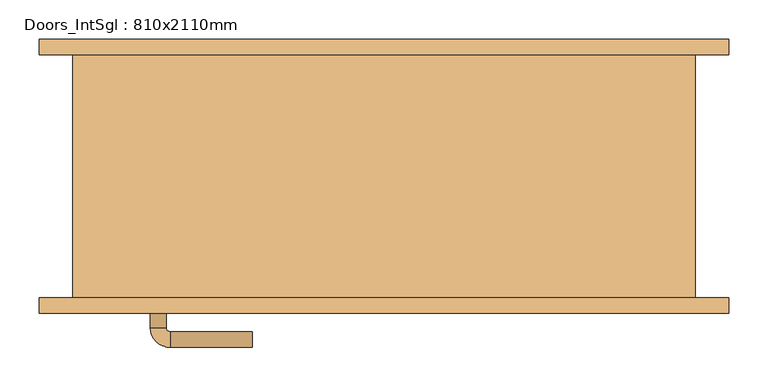
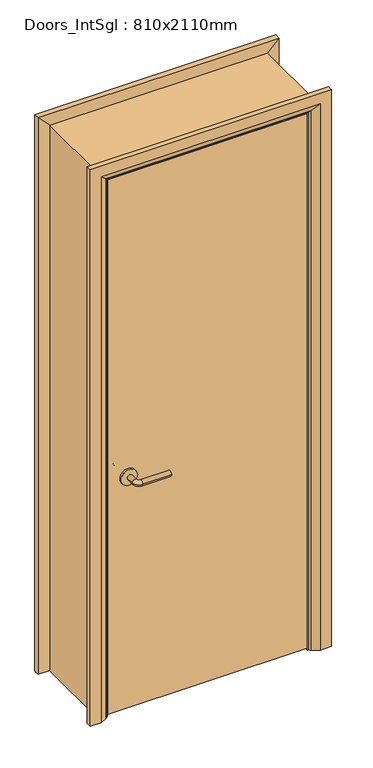
"""IFC4 building model written with IfcOpenShell, lengths in millimetres: door geometry, Doors_IntSgl : 810x2110mm."""

from ifc_helpers import new_model, si_unit, point, frame, frame_2d, origin, place, context, project, spatial, polyline, circle_curve, ellipse_curve, trimmed, segment, composite_curve, outline, extrude, faceted_brep, source, transform, mapped, element, save
from ifc_brep_helpers import plane_surface, cylinder_surface, revolved_surface, advanced_brep


def doors_intsgl_810x2110mm_eeb1298a(model_context):
    return source(origin(), model_context, "Body", "SolidModel", [
        advanced_brep(
        [(-298.0, -109.0, 900.0), (-278.0, -109.0, 900.0), (-298.0, -79.0, 900.0), (-278.0, -79.0, 900.0), (-273.0, -74.0, 900.0), (-273.0, -54.0, 900.0), (-168.0, -54.0, 900.0), (-168.0, -74.0, 900.0)],
        [
            (0, 1, circle_curve(frame((-288.0, -109.0, 900.0), z_axis=(0.0, -1.0, 0.0), x_axis=(1.0, 0.0, 0.0)), 10.0)),
            (1, 0, circle_curve(frame((-288.0, -109.0, 900.0), z_axis=(0.0, -1.0, 0.0), x_axis=(1.0, 0.0, 0.0)), 10.0)),
            (0, 2),
            (2, 3, circle_curve(frame((-288.0, -79.0, 900.0), z_axis=(0.0, -1.0, 0.0), x_axis=(1.0, 0.0, 0.0)), 10.0)),
            (3, 1),
            (3, 2, circle_curve(frame((-288.0, -79.0, 900.0), z_axis=(0.0, -1.0, 0.0), x_axis=(1.0, 0.0, 0.0)), 10.0)),
            (4, 3, circle_curve(frame((-273.0, -79.0, 900.0), z_axis=(0.0, 0.0, 1.0), x_axis=(-1.0, 0.0, 0.0)), 5.0)),
            (2, 5, circle_curve(frame((-273.0, -79.0, 900.0), z_axis=(0.0, 0.0, -1.0), x_axis=(-1.0, 0.0, 0.0)), 25.0)),
            (5, 4, circle_curve(frame((-273.0, -64.0, 900.0), z_axis=(-1.0, 0.0, 0.0), x_axis=(0.0, -1.0, 0.0)), 10.0)),
            (4, 5, circle_curve(frame((-273.0, -64.0, 900.0), z_axis=(-1.0, 0.0, 0.0), x_axis=(0.0, -1.0, 0.0)), 10.0)),
            (6, 7, circle_curve(frame((-168.0, -64.0, 900.0), z_axis=(1.0, 0.0, 0.0), x_axis=(0.0, -1.0, 0.0)), 10.0)),
            (7, 6, circle_curve(frame((-168.0, -64.0, 900.0), z_axis=(1.0, 0.0, 0.0), x_axis=(0.0, -1.0, 0.0)), 10.0)),
            (5, 6),
            (7, 4),
        ],
        [
            plane_surface(frame((-288.0, -109.0, 900.0), z_axis=(0.0, -1.0, 0.0), x_axis=(0.0, 0.0, 1.0))),
            cylinder_surface(frame((-288.0, -109.0, 900.0), z_axis=(0.0, -1.0, 0.0), x_axis=(1.0, 0.0, 0.0)), 10.0),
            revolved_surface(trimmed(ellipse_curve(frame((-288.0, -79.0, 900.0), z_axis=(0.0, -1.0, 0.0), x_axis=(1.0, 0.0, 0.0)), 10.0, 10.0), [point((-298.0, -79.0, 900.0))], [point((-278.0, -79.0, 900.0))], True, "CARTESIAN"), (-273.0, -79.0, 900.0), (0.0, 0.0, -1.0)),
            revolved_surface(trimmed(ellipse_curve(frame((-288.0, -79.0, 900.0), z_axis=(0.0, -1.0, 0.0), x_axis=(1.0, 0.0, 0.0)), 10.0, 10.0), [point((-278.0, -79.0, 900.0))], [point((-298.0, -79.0, 900.0))], True, "CARTESIAN"), (-273.0, -79.0, 900.0), (0.0, 0.0, -1.0)),
            plane_surface(frame((-168.0, -64.0, 900.0), z_axis=(1.0, 0.0, 0.0), x_axis=(0.0, 0.0, 1.0))),
            cylinder_surface(frame((-273.0, -64.0, 900.0), z_axis=(-1.0, 0.0, 0.0), x_axis=(0.0, -1.0, 0.0)), 10.0),
        ],
        [
            (0, [[1, 2]]),
            (1, [[-1, 3, 4, 5]]),
            (1, [[-2, -5, 6, -3]]),
            (2, [[7, -4, 8, 9]]),
            (3, [[-8, -6, -7, 10]]),
            (4, [[11, 12]]),
            (5, [[-9, 13, -12, 14]]),
            (5, [[-10, -14, -11, -13]]),
        ],
    ),
        extrude(outline(composite_curve([segment(trimmed(circle_curve(frame_2d((900.0, -290.5)), 30.0), [point((900.0, -320.5))], [point((900.0, -260.5))], False, "CARTESIAN"), True, "CONTINUOUS"), segment(trimmed(circle_curve(frame_2d((900.0, -290.5)), 30.0), [point((900.0, -260.5))], [point((900.0, -320.5))], False, "CARTESIAN"), True, "CONTINUOUS")], self_intersect=False)), frame((0.0, -117.0, 0.0), z_axis=(0.0, 1.0, 0.0), x_axis=(0.0, 0.0, 1.0)), (0.0, 0.0, 1.0), 8.0),
        advanced_brep(
        [(-298.0, -163.0, 900.0), (-278.0, -163.0, 900.0), (-278.0, -193.0, 900.0), (-298.0, -193.0, 900.0), (-273.0, -198.0, 900.0), (-273.0, -218.0, 900.0), (-168.0, -218.0, 900.0), (-168.0, -198.0, 900.0)],
        [
            (0, 1, circle_curve(frame((-288.0, -163.0, 900.0), z_axis=(0.0, 1.0, 0.0), x_axis=(1.0, 0.0, 0.0)), 10.0)),
            (1, 0, circle_curve(frame((-288.0, -163.0, 900.0), z_axis=(0.0, 1.0, 0.0), x_axis=(1.0, 0.0, 0.0)), 10.0)),
            (1, 2),
            (2, 3, circle_curve(frame((-288.0, -193.0, 900.0), z_axis=(0.0, 1.0, 0.0), x_axis=(1.0, 0.0, 0.0)), 10.0)),
            (3, 0),
            (3, 2, circle_curve(frame((-288.0, -193.0, 900.0), z_axis=(0.0, 1.0, 0.0), x_axis=(1.0, 0.0, 0.0)), 10.0)),
            (4, 5, circle_curve(frame((-273.0, -208.0, 900.0), z_axis=(-1.0, 0.0, 0.0), x_axis=(0.0, 1.0, 0.0)), 10.0)),
            (5, 3, circle_curve(frame((-273.0, -193.0, 900.0), z_axis=(0.0, 0.0, -1.0), x_axis=(-1.0, 0.0, 0.0)), 25.0)),
            (2, 4, circle_curve(frame((-273.0, -193.0, 900.0), z_axis=(0.0, 0.0, 1.0), x_axis=(-1.0, 0.0, 0.0)), 5.0)),
            (5, 4, circle_curve(frame((-273.0, -208.0, 900.0), z_axis=(-1.0, 0.0, 0.0), x_axis=(0.0, 1.0, 0.0)), 10.0)),
            (6, 7, circle_curve(frame((-168.0, -208.0, 900.0), z_axis=(1.0, 0.0, 0.0), x_axis=(0.0, 1.0, 0.0)), 10.0)),
            (7, 6, circle_curve(frame((-168.0, -208.0, 900.0), z_axis=(1.0, 0.0, 0.0), x_axis=(0.0, 1.0, 0.0)), 10.0)),
            (4, 7),
            (6, 5),
        ],
        [
            plane_surface(frame((-288.0, -163.0, 900.0), z_axis=(0.0, 1.0, 0.0), x_axis=(0.0, 0.0, 1.0))),
            cylinder_surface(frame((-288.0, -163.0, 900.0), z_axis=(0.0, 1.0, 0.0), x_axis=(1.0, 0.0, 0.0)), 10.0),
            revolved_surface(trimmed(ellipse_curve(frame((-288.0, -193.0, 900.0), z_axis=(0.0, -1.0, 0.0), x_axis=(1.0, 0.0, 0.0)), 10.0, 10.0), [point((-298.0, -193.0, 900.0))], [point((-278.0, -193.0, 900.0))], True, "CARTESIAN"), (-273.0, -193.0, 900.0), (0.0, 0.0, -1.0)),
            revolved_surface(trimmed(ellipse_curve(frame((-288.0, -193.0, 900.0), z_axis=(0.0, -1.0, 0.0), x_axis=(1.0, 0.0, 0.0)), 10.0, 10.0), [point((-278.0, -193.0, 900.0))], [point((-298.0, -193.0, 900.0))], True, "CARTESIAN"), (-273.0, -193.0, 900.0), (0.0, 0.0, -1.0)),
            plane_surface(frame((-168.0, -208.0, 900.0), z_axis=(1.0, 0.0, 0.0), x_axis=(0.0, 0.0, 1.0))),
            cylinder_surface(frame((-273.0, -208.0, 900.0), z_axis=(-1.0, 0.0, 0.0), x_axis=(0.0, 1.0, 0.0)), 10.0),
        ],
        [
            (0, [[1, 2]]),
            (1, [[3, 4, 5, -2]]),
            (1, [[-5, 6, -3, -1]]),
            (2, [[7, 8, -4, 9]]),
            (3, [[10, -9, -6, -8]]),
            (4, [[11, 12]]),
            (5, [[13, -11, 14, -7]]),
            (5, [[-14, -12, -13, -10]]),
        ],
    ),
        extrude(outline(composite_curve([segment(trimmed(circle_curve(frame_2d((900.0, -290.5)), 30.0), [point((900.0, -320.5))], [point((900.0, -260.5))], False, "CARTESIAN"), True, "CONTINUOUS"), segment(trimmed(circle_curve(frame_2d((900.0, -290.5)), 30.0), [point((900.0, -260.5))], [point((900.0, -320.5))], False, "CARTESIAN"), True, "CONTINUOUS")], self_intersect=False)), frame((0.0, -163.0, 0.0), z_axis=(0.0, 1.0, 0.0), x_axis=(0.0, 0.0, 1.0)), (0.0, 0.0, 1.0), 8.0),
        extrude(outline(polyline([(363.0, -117.0), (363.0, -155.0), (-363.0, -155.0), (-363.0, -117.0), (363.0, -117.0)])), frame((0.0, 0.0, 8.0), z_axis=(0.0, 0.0, 1.0), x_axis=(1.0, 0.0, 0.0)), (0.0, 0.0, 1.0), 2060.0),
        advanced_brep(
        [(440.0, -175.0, 0.0), (400.0, -175.0, 0.0), (374.0, -161.0, 0.0), (370.0, -155.0, 0.0), (440.0, -155.0, 0.0), (440.0, -155.0, 2145.0), (440.0, -175.0, 2145.0), (370.0, -155.0, 2075.0), (-370.0, -155.0, 2075.0), (-370.0, -155.0, 0.0), (-440.0, -155.0, 0.0), (-440.0, -155.0, 2145.0), (374.0, -161.0, 2079.0), (400.0, -175.0, 2105.0), (-440.0, -175.0, 2145.0), (-440.0, -175.0, 0.0), (-400.0, -175.0, 0.0), (-400.0, -175.0, 2105.0), (-374.0, -161.0, 2079.0), (-374.0, -161.0, 0.0)],
        [
            (0, 1),
            (1, 2),
            (2, 3, circle_curve(frame((378.0, -154.0, 0.0), z_axis=(0.0, 0.0, -1.0), x_axis=(1.0, 0.0, 0.0)), 8.0622577)),
            (3, 4),
            (4, 0),
            (4, 5),
            (5, 6),
            (6, 0),
            (3, 7),
            (7, 8),
            (8, 9),
            (9, 10),
            (10, 11),
            (11, 5),
            (2, 12),
            (12, 7, ellipse_curve(frame((378.0, -154.0, 2083.0), z_axis=(0.7071067811865475, 0.0, -0.7071067811865475), x_axis=(-0.7071067811865474, 0.0, -0.7071067811865476)), 11.4017543, 8.0622577)),
            (1, 13),
            (13, 12),
            (6, 14),
            (14, 15),
            (15, 16),
            (16, 17),
            (17, 13),
            (11, 14),
            (12, 18),
            (18, 8, ellipse_curve(frame((-378.0, -154.0, 2083.0), z_axis=(0.7071067811865475, 0.0, 0.7071067811865475), x_axis=(0.7071067811865476, 0.0, -0.7071067811865474)), 11.4017543, 8.0622577)),
            (17, 18),
            (15, 10),
            (9, 19, circle_curve(frame((-378.0, -154.0, 0.0), z_axis=(0.0, 0.0, -1.0), x_axis=(-1.0, 0.0, 0.0)), 8.0622577)),
            (19, 16),
            (18, 19),
        ],
        [
            plane_surface(frame((370.0, -155.0, 0.0), z_axis=(0.0, 0.0, -1.0), x_axis=(0.0, 1.0, 0.0))),
            plane_surface(frame((440.0, -175.0, 0.0), z_axis=(1.0, 0.0, 0.0), x_axis=(0.0, 0.0, 1.0))),
            plane_surface(frame((440.0, -155.0, 0.0), z_axis=(0.0, 1.0, 0.0), x_axis=(0.0, 0.0, 1.0))),
            cylinder_surface(frame((378.0, -154.0, 0.0), z_axis=(0.0, 0.0, -1.0), x_axis=(1.0, 0.0, 0.0)), 8.0622577),
            plane_surface(frame((374.0, -161.0, 0.0), z_axis=(-0.4740998230350126, -0.880471099922178, 0.0), x_axis=(0.0, 0.0, 1.0))),
            plane_surface(frame((400.0, -175.0, 0.0), z_axis=(0.0, -1.0, 0.0), x_axis=(0.0, 0.0, 1.0))),
            plane_surface(frame((440.0, -175.0, 2145.0), z_axis=(0.0, 0.0, 1.0), x_axis=(-1.0, 0.0, 0.0))),
            cylinder_surface(frame((370.0, -154.0, 2083.0), z_axis=(1.0, 0.0, 0.0), x_axis=(0.0, 0.0, 1.0)), 8.0622577),
            plane_surface(frame((374.0, -161.0, 2079.0), z_axis=(0.0, -0.8804710999221764, -0.4740998230350154), x_axis=(-1.0, 0.0, 0.0))),
            plane_surface(frame((-370.0, -155.0, 0.0), z_axis=(0.0, 0.0, -1.0), x_axis=(0.0, 1.0, 0.0))),
            plane_surface(frame((-440.0, -175.0, 2145.0), z_axis=(-1.0, 0.0, 0.0), x_axis=(0.0, 0.0, -1.0))),
            cylinder_surface(frame((-378.0, -154.0, 2075.0), z_axis=(0.0, 0.0, 1.0), x_axis=(-1.0, 0.0, 0.0)), 8.0622577),
            plane_surface(frame((-374.0, -161.0, 2079.0), z_axis=(0.47409982303501824, -0.8804710999221749, 0.0), x_axis=(0.0, 0.0, -1.0))),
        ],
        [
            (0, [[1, 2, 3, 4, 5]]),
            (1, [[6, 7, 8, -5]]),
            (2, [[9, 10, 11, 12, 13, 14, -6, -4]]),
            (3, [[15, 16, -9, -3]]),
            (4, [[17, 18, -15, -2]]),
            (5, [[-8, 19, 20, 21, 22, 23, -17, -1]]),
            (6, [[-14, 24, -19, -7]]),
            (7, [[25, 26, -10, -16]]),
            (8, [[-23, 27, -25, -18]]),
            (9, [[28, -12, 29, 30, -21]]),
            (10, [[-13, -28, -20, -24]]),
            (11, [[31, -29, -11, -26]]),
            (12, [[-22, -30, -31, -27]]),
        ],
    ),
        extrude(outline(polyline([(0.0, -346.0), (2051.0, -346.0), (2051.0, 346.0), (0.0, 346.0), (0.0, 365.0), (2070.0, 365.0), (2070.0, -365.0), (0.0, -365.0), (0.0, -346.0)])), frame((0.0, -115.0, 0.0), z_axis=(0.0, 1.0, 0.0), x_axis=(0.0, 0.0, 1.0)), (0.0, 0.0, 1.0), 32.0),
        advanced_brep(
        [(-440.0, 175.0, 0.0), (-400.0, 175.0, 0.0), (-374.0, 161.0, 0.0), (-370.0, 155.0, 0.0), (-440.0, 155.0, 0.0), (-440.0, 155.0, 2145.0), (-440.0, 175.0, 2145.0), (-370.0, 155.0, 2075.0), (-374.0, 161.0, 2079.0), (-400.0, 175.0, 2105.0), (440.0, 155.0, 2145.0), (440.0, 175.0, 2145.0), (370.0, 155.0, 2075.0), (374.0, 161.0, 2079.0), (400.0, 175.0, 2105.0), (440.0, 175.0, 0.0), (440.0, 155.0, 0.0), (370.0, 155.0, 0.0), (374.0, 161.0, 0.0), (400.0, 175.0, 0.0)],
        [
            (0, 1),
            (1, 2),
            (2, 3, circle_curve(frame((-378.0, 154.0, 0.0), z_axis=(0.0, 0.0, -1.0), x_axis=(-1.0, 0.0, 0.0)), 8.0622577)),
            (3, 4),
            (4, 0),
            (4, 5),
            (5, 6),
            (6, 0),
            (3, 7),
            (7, 5),
            (2, 8),
            (8, 7, ellipse_curve(frame((-378.0, 154.0, 2083.0), z_axis=(-0.7071067811865475, 0.0, -0.7071067811865475), x_axis=(0.7071067811865474, 0.0, -0.7071067811865476)), 11.4017543, 8.0622577)),
            (1, 9),
            (9, 8),
            (6, 9),
            (5, 10),
            (10, 11),
            (11, 6),
            (7, 12),
            (12, 10),
            (8, 13),
            (13, 12, ellipse_curve(frame((378.0, 154.0, 2083.0), z_axis=(-0.7071067811865475, 0.0, 0.7071067811865475), x_axis=(-0.7071067811865476, 0.0, -0.7071067811865474)), 11.4017543, 8.0622577)),
            (9, 14),
            (14, 13),
            (11, 14),
            (15, 16),
            (16, 17),
            (17, 18, circle_curve(frame((378.0, 154.0, 0.0), z_axis=(0.0, 0.0, -1.0), x_axis=(1.0, 0.0, 0.0)), 8.0622577)),
            (18, 19),
            (19, 15),
            (10, 16),
            (15, 11),
            (12, 17),
            (13, 18),
            (14, 19),
        ],
        [
            plane_surface(frame((-370.0, 227.8010989, 0.0), z_axis=(0.0, 0.0, -1.0), x_axis=(1.0, 0.0, 0.0))),
            plane_surface(frame((-440.0, 175.0, 0.0), z_axis=(-1.0, 0.0, 0.0), x_axis=(0.0, 0.0, 1.0))),
            plane_surface(frame((-440.0, 155.0, 0.0), z_axis=(0.0, -1.0, 0.0), x_axis=(0.0, 0.0, 1.0))),
            cylinder_surface(frame((-378.0, 154.0, 0.0), z_axis=(0.0, 0.0, -1.0), x_axis=(-1.0, 0.0, 0.0)), 8.0622577),
            plane_surface(frame((-374.0, 161.0, 0.0), z_axis=(0.4740998230350183, 0.8804710999221749, 0.0), x_axis=(0.0, 0.0, 1.0))),
            plane_surface(frame((-400.0, 175.0, 0.0), z_axis=(0.0, 1.0, 0.0), x_axis=(0.0, 0.0, 1.0))),
            plane_surface(frame((-440.0, 175.0, 2145.0), z_axis=(0.0, 0.0, 1.0), x_axis=(1.0, 0.0, 0.0))),
            plane_surface(frame((-440.0, 155.0, 2145.0), z_axis=(0.0, -1.0, 0.0), x_axis=(1.0, 0.0, 0.0))),
            cylinder_surface(frame((-370.0, 154.0, 2083.0), z_axis=(-1.0, 0.0, 0.0), x_axis=(0.0, 0.0, 1.0)), 8.0622577),
            plane_surface(frame((-374.0, 161.0, 2079.0), z_axis=(0.0, 0.8804710999221749, -0.4740998230350183), x_axis=(1.0, 0.0, 0.0))),
            plane_surface(frame((-400.0, 175.0, 2105.0), z_axis=(0.0, 1.0, 0.0), x_axis=(1.0, 0.0, 0.0))),
            plane_surface(frame((370.0, 227.8010989, 0.0), z_axis=(0.0, 0.0, -1.0), x_axis=(-1.0, 0.0, 0.0))),
            plane_surface(frame((440.0, 175.0, 2145.0), z_axis=(1.0, 0.0, 0.0), x_axis=(0.0, 0.0, -1.0))),
            plane_surface(frame((440.0, 155.0, 2145.0), z_axis=(0.0, -1.0, 0.0), x_axis=(0.0, 0.0, -1.0))),
            cylinder_surface(frame((378.0, 154.0, 2075.0), z_axis=(0.0, 0.0, 1.0), x_axis=(1.0, 0.0, 0.0)), 8.0622577),
            plane_surface(frame((374.0, 161.0, 2079.0), z_axis=(-0.4740998230350183, 0.8804710999221749, 0.0), x_axis=(0.0, 0.0, -1.0))),
            plane_surface(frame((400.0, 175.0, 2105.0), z_axis=(0.0, 1.0, 0.0), x_axis=(0.0, 0.0, -1.0))),
        ],
        [
            (0, [[1, 2, 3, 4, 5]]),
            (1, [[6, 7, 8, -5]]),
            (2, [[9, 10, -6, -4]]),
            (3, [[11, 12, -9, -3]]),
            (4, [[13, 14, -11, -2]]),
            (5, [[-8, 15, -13, -1]]),
            (6, [[16, 17, 18, -7]]),
            (7, [[19, 20, -16, -10]]),
            (8, [[21, 22, -19, -12]]),
            (9, [[23, 24, -21, -14]]),
            (10, [[-18, 25, -23, -15]]),
            (11, [[26, 27, 28, 29, 30]]),
            (12, [[31, -26, 32, -17]]),
            (13, [[33, -27, -31, -20]]),
            (14, [[34, -28, -33, -22]]),
            (15, [[35, -29, -34, -24]]),
            (16, [[-32, -30, -35, -25]]),
        ],
    ),
        faceted_brep([(-365.0, -155.0, 0.0), (-397.0, -155.0, 0.0), (-397.0, 155.0, 0.0), (-365.0, 155.0, 0.0), (-365.0, 155.0, 2070.0), (-365.0, -155.0, 2070.0), (-397.0, 155.0, 2102.0), (-397.0, -155.0, 2102.0), (365.0, 155.0, 2070.0), (365.0, -155.0, 2070.0), (397.0, 155.0, 2102.0), (397.0, -155.0, 2102.0), (365.0, -155.0, 0.0), (365.0, 155.0, 0.0), (397.0, 155.0, 0.0), (397.0, -155.0, 0.0)], [[[0, 1, 2, 3]], [[3, 4, 5, 0]], [[2, 6, 4, 3]], [[1, 7, 6, 2]], [[0, 5, 7, 1]], [[4, 8, 9, 5]], [[6, 10, 8, 4]], [[7, 11, 10, 6]], [[5, 9, 11, 7]], [[12, 13, 14, 15]], [[8, 13, 12, 9]], [[10, 14, 13, 8]], [[11, 15, 14, 10]], [[9, 12, 15, 11]]]),
    ])


if __name__ == "__main__":
    model = new_model("IFC4")
    model_context = context("Model", 3, world=origin())
    ifc_project = project(units=[si_unit("LENGTHUNIT", "METRE", prefix="MILLI")], contexts=[model_context])
    site = spatial("IfcSite", under=ifc_project)
    building = spatial("IfcBuilding", under=site)
    placement = place(None, origin())
    doors_intsgl_810x2110mm_shape = doors_intsgl_810x2110mm_eeb1298a(model_context)
    element("IfcDoor", 1, ObjectType="Doors_IntSgl : 810x2110mm", at=placement, inside=building, context=model_context, shape_type="MappedRepresentation", body=[
        mapped(doors_intsgl_810x2110mm_shape, transform((0.0, 0.0, 0.0), x_axis=(1.0, 0.0, 0.0), y_axis=(0.0, 1.0, 0.0), z_axis=(0.0, 0.0, 1.0))),
    ])
    save(model, "model.ifc")

# Revit data of these elements
# Type "Doors_IntSgl : 810x2110mm"
#   Construction Type Id = "MDOOR"
#   Type Mark = "42"
#   Type Comments = "Internal Single"
#   Operation = "SingleSwingRight"
#   Manufacturer = "Revit"
#   Keynote = "L20"
#   Description = "Internal Single Door"
#   Analytic Construction = "Metal"
#   UnderCut = 8 mm
#   Tolerance = 2 mm
#   Thickness = 38 mm
#   Thermal Resistance (R) = 0.270117 (m²·K)/W
#   Structural Tolerance = 8 mm
#   StopDepth = 32 mm
#   Stop Thickness = 19 mm
#   Rough Width = 810 mm
#   Rough Height = 2110 mm
#   Height to Top Lock Rail = 1000 mm
#   Heat Transfer Coefficient (U) = 3.7021 W/(m²·K)
#   Handle Z Distance = 900 mm
#   Handle X Distance = 75 mm
#   Frame Thickness = 32 mm
#   Door Panel Width = 726 mm
#   Door Panel Thickness = 38 mm
#   Door Panel Offset = 0 mm
#   Height = 2110 mm
#   Width = 810 mm
#   Door Panel Height = 2060 mm
#   Architrave Setback = 5 mm
#   Define Thermal Properties by = 1
#   Vis - Ironmongery = yes
#   Material Ironmongery = Door - Handle
#   Material Frame = Door - Frame/Mullion (1)
#   Material Door = Door - Panel
#   Material Architrave = Door - Architrave
#   Visual Light Transmittance = 0
#   Solar Heat Gain Coefficient = 0
#   Function = (empty or 0)
#   Wall Closure = (empty or 0)
# Element 1 (IfcDoor, "Doors_IntSgl : 810x2110mm")
#   Materials on its faces: "Door - Architrave", "Door - Handle", "Door - Frame/Mullion (1)", "Door - Panel"
# Materials
#   "Door - Handle": class "Miscellaneous", colour RGB 0 0 0, transparency 0, Keynote = "P21", Cost = 0
#   "Door - Frame/Mullion (1)": class "Wood", colour RGB 212 179 113, transparency 0, Keynote = "L20", Cost = 0
#   "Door - Panel": class "Wood", colour RGB 210 159 95, transparency 0, Keynote = "L20", Cost = 0
#   "Door - Architrave": class "Wood", colour RGB 154 90 5, transparency 0, Keynote = "P20", Cost = 0
